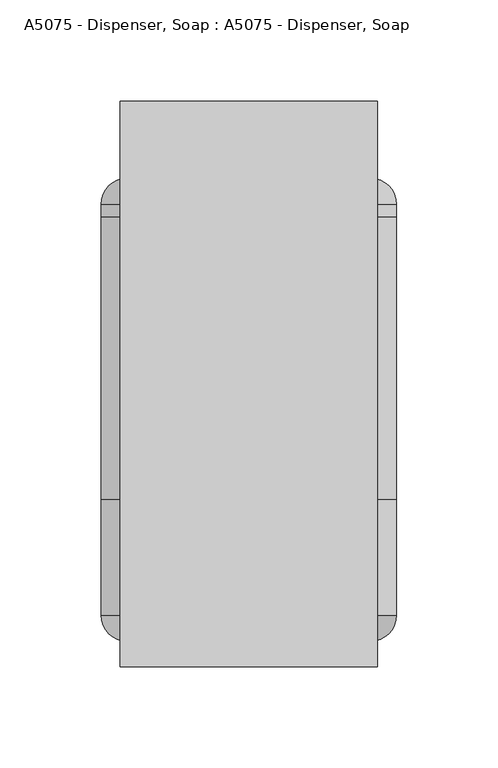
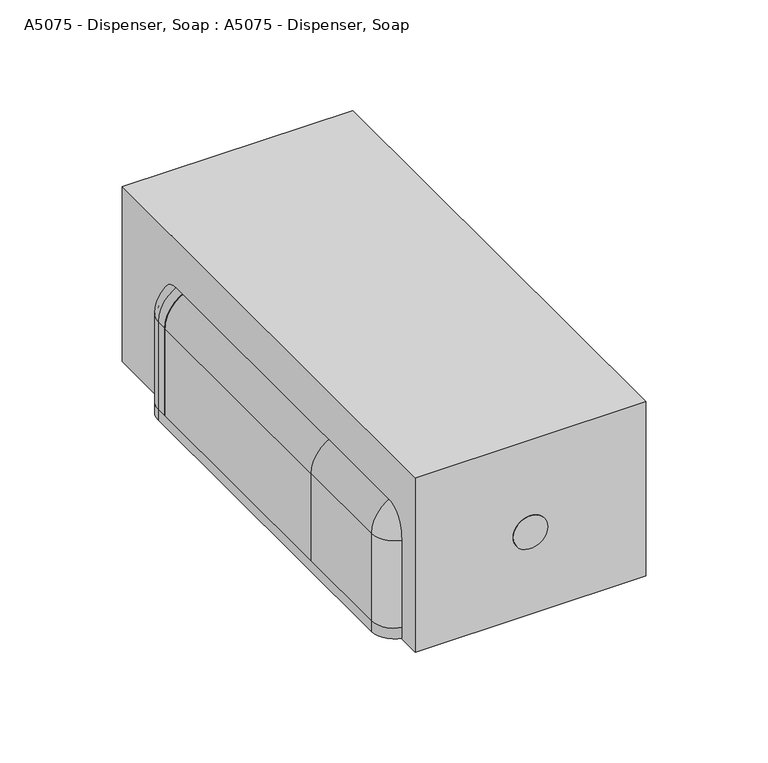
"""IFC4 building model written with IfcOpenShell, lengths in millimetres: proxy geometry, A5075 - Dispenser, Soap : A5075 - Dispenser, Soap."""

from ifc_helpers import new_model, si_unit, point, frame, frame_2d, origin, origin_with_axes, place, context, project, spatial, polyline, circle_curve, ellipse_curve, trimmed, segment, composite_curve, outline, extrude, source, transform, mapped, element, save
from ifc_brep_helpers import plane_surface, cylinder_surface, revolved_surface, advanced_brep


def a5075_dispenser_soap_a5075_dispenser_soap_4b3b6f7a(model_context):
    return source(origin(), model_context, "Body", "SolidModel", [
        advanced_brep(
        [(-73.025, 25.4, 6.35), (-73.025, 82.55, 6.35), (-71.4375, 82.55, 6.35), (-71.4375, 25.4, 6.35), (-60.325, 14.2875, 6.35), (-60.325, 12.7, 6.35), (-73.025, 25.4, 57.15), (-73.025, 82.55, 57.15), (-53.975, 82.55, 76.2), (53.975, 82.55, 76.2), (73.025, 82.55, 57.15), (73.025, 82.55, 6.35), (71.4375, 82.55, 6.35), (71.4375, 82.55, 57.15), (53.975, 82.55, 74.6125), (-53.975, 82.55, 74.6125), (-71.4375, 82.55, 57.15), (-71.4375, 25.4, 57.15), (-60.325, 14.2875, 57.15), (-60.325, 12.7, 57.15), (-53.975, 25.4, 76.2), (-53.975, 25.4, 74.6125), (-53.975, 14.2875, 63.5), (-53.975, 12.7, 63.5), (53.975, 25.4, 76.2), (53.975, 25.4, 74.6125), (53.975, 14.2875, 63.5), (53.975, 12.7, 63.5), (73.025, 25.4, 57.15), (71.4375, 25.4, 57.15), (60.325, 14.2875, 57.15), (60.325, 12.7, 57.15), (73.025, 25.4, 6.35), (60.325, 12.7, 6.35), (60.325, 14.2875, 6.35), (71.4375, 25.4, 6.35)],
        [
            (0, 1),
            (1, 2),
            (2, 3),
            (3, 4, circle_curve(frame((-60.325, 25.4, 6.35), z_axis=(0.0, 0.0, 1.0), x_axis=(1.0, 0.0, 0.0)), 11.1125)),
            (4, 5),
            (5, 0, circle_curve(frame((-60.325, 25.4, 6.35), z_axis=(0.0, 0.0, -1.0), x_axis=(1.0, 0.0, 0.0)), 12.7)),
            (0, 6),
            (6, 7),
            (7, 1),
            (7, 8, circle_curve(frame((-53.975, 82.55, 57.15), z_axis=(0.0, 1.0, 0.0), x_axis=(-1.0, 0.0, 0.0)), 19.05)),
            (8, 9),
            (9, 10, circle_curve(frame((53.975, 82.55, 57.15), z_axis=(0.0, 1.0, 0.0), x_axis=(0.0, 0.0, 1.0)), 19.05)),
            (10, 11),
            (11, 12),
            (12, 13),
            (13, 14, circle_curve(frame((53.975, 82.55, 57.15), z_axis=(0.0, -1.0, 0.0), x_axis=(0.0, 0.0, 1.0)), 17.4625)),
            (14, 15),
            (15, 16, circle_curve(frame((-53.975, 82.55, 57.15), z_axis=(0.0, -1.0, 0.0), x_axis=(-1.0, 0.0, 0.0)), 17.4625)),
            (16, 2),
            (16, 17),
            (17, 3),
            (17, 18, circle_curve(frame((-60.325, 25.4, 57.15), z_axis=(0.0, 0.0, 1.0), x_axis=(1.0, 0.0, 0.0)), 11.1125)),
            (18, 4),
            (18, 19),
            (19, 5),
            (19, 6, circle_curve(frame((-60.325, 25.4, 57.15), z_axis=(0.0, 0.0, -1.0), x_axis=(1.0, 0.0, 0.0)), 12.7)),
            (6, 20, circle_curve(frame((-53.975, 25.4, 57.15), z_axis=(0.0, 1.0, 0.0), x_axis=(-1.0, 0.0, 0.0)), 19.05)),
            (20, 8),
            (21, 17, circle_curve(frame((-53.975, 25.4, 57.15), z_axis=(0.0, -1.0, 0.0), x_axis=(-1.0, 0.0, 0.0)), 17.4625)),
            (15, 21),
            (22, 18, circle_curve(frame((-53.975, 14.2875, 57.15), z_axis=(0.0, -1.0, 0.0), x_axis=(-1.0, 0.0, 0.0)), 6.35)),
            (21, 22, circle_curve(frame((-53.975, 25.4, 63.5), z_axis=(1.0, 0.0, 0.0), x_axis=(0.0, 0.0, -1.0)), 11.1125)),
            (23, 19, circle_curve(frame((-53.975, 12.7, 57.15), z_axis=(0.0, -1.0, 0.0), x_axis=(-1.0, 0.0, 0.0)), 6.35)),
            (22, 23),
            (23, 20, circle_curve(frame((-53.975, 25.4, 63.5), z_axis=(-1.0, 0.0, 0.0), x_axis=(0.0, 0.0, -1.0)), 12.7)),
            (20, 24),
            (24, 9),
            (14, 25),
            (25, 21),
            (25, 26, circle_curve(frame((53.975, 25.4, 63.5), z_axis=(1.0, 0.0, 0.0), x_axis=(0.0, 0.0, -1.0)), 11.1125)),
            (26, 22),
            (26, 27),
            (27, 23),
            (27, 24, circle_curve(frame((53.975, 25.4, 63.5), z_axis=(-1.0, 0.0, 0.0), x_axis=(0.0, 0.0, -1.0)), 12.7)),
            (24, 28, circle_curve(frame((53.975, 25.4, 57.15), z_axis=(0.0, 1.0, 0.0), x_axis=(0.0, 0.0, 1.0)), 19.05)),
            (28, 10),
            (29, 25, circle_curve(frame((53.975, 25.4, 57.15), z_axis=(0.0, -1.0, 0.0), x_axis=(0.0, 0.0, 1.0)), 17.4625)),
            (13, 29),
            (30, 26, circle_curve(frame((53.975, 14.2875, 57.15), z_axis=(0.0, -1.0, 0.0), x_axis=(0.0, 0.0, 1.0)), 6.35)),
            (29, 30, circle_curve(frame((60.325, 25.4, 57.15), z_axis=(0.0, 0.0, -1.0), x_axis=(-1.0, 0.0, 0.0)), 11.1125)),
            (31, 27, circle_curve(frame((53.975, 12.7, 57.15), z_axis=(0.0, -1.0, 0.0), x_axis=(0.0, 0.0, 1.0)), 6.35)),
            (30, 31),
            (31, 28, circle_curve(frame((60.325, 25.4, 57.15), z_axis=(0.0, 0.0, 1.0), x_axis=(-1.0, 0.0, 0.0)), 12.7)),
            (32, 33, circle_curve(frame((60.325, 25.4, 6.35), z_axis=(0.0, 0.0, -1.0), x_axis=(-1.0, 0.0, 0.0)), 12.7)),
            (33, 34),
            (34, 35, circle_curve(frame((60.325, 25.4, 6.35), z_axis=(0.0, 0.0, 1.0), x_axis=(-1.0, 0.0, 0.0)), 11.1125)),
            (35, 12),
            (11, 32),
            (28, 32),
            (35, 29),
            (34, 30),
            (33, 31),
        ],
        [
            plane_surface(frame((-73.025, 12.7, 6.35), z_axis=(0.0, 0.0, -1.0), x_axis=(0.0, 1.0, 0.0))),
            plane_surface(frame((-73.025, 25.4, 6.35), z_axis=(-1.0, 0.0, 0.0), x_axis=(0.0, 0.0, 1.0))),
            plane_surface(frame((-73.025, 82.55, 6.35), z_axis=(0.0, 1.0, 0.0), x_axis=(0.0, 0.0, 1.0))),
            plane_surface(frame((-71.4375, 82.55, 6.35), z_axis=(1.0, 0.0, 0.0), x_axis=(0.0, 0.0, 1.0))),
            revolved_surface(polyline([(-49.212500000000006, 25.4, 57.15), (-49.212500000000006, 25.4, 6.35)]), (-60.325, 25.4, 6.35), (0.0, 0.0, 1.0)),
            plane_surface(frame((-60.325, 14.2875, 6.35), z_axis=(1.0, 0.0, 0.0), x_axis=(0.0, 0.0, 1.0))),
            cylinder_surface(frame((-60.325, 25.4, 6.35), z_axis=(0.0, 0.0, -1.0), x_axis=(1.0, 0.0, 0.0)), 12.7),
            cylinder_surface(frame((-53.975, 12.7, 57.15), z_axis=(0.0, 1.0, 0.0), x_axis=(-1.0, 0.0, 0.0)), 19.05),
            revolved_surface(polyline([(-71.4375, 82.55, 57.15), (-71.4375, 25.4, 57.15)]), (-53.975, 12.7, 57.15), (0.0, 1.0, 0.0)),
            revolved_surface(trimmed(ellipse_curve(frame((-60.325, 25.4, 57.15), z_axis=(0.0, 0.0, 1.0), x_axis=(1.0, 0.0, 0.0)), 11.1125, 11.1125), [point((-71.4375, 25.4, 57.15))], [point((-60.325, 14.2875, 57.15))], True, "CARTESIAN"), (-53.975, 12.7, 57.15), (0.0, 1.0, 0.0)),
            revolved_surface(polyline([(-60.325, 14.2875, 57.15), (-60.325, 12.7, 57.15)]), (-53.975, 12.7, 57.15), (0.0, 1.0, 0.0)),
            revolved_surface(trimmed(ellipse_curve(frame((-60.325, 25.4, 57.15), z_axis=(0.0, 0.0, -1.0), x_axis=(1.0, 0.0, 0.0)), 12.7, 12.7), [point((-60.325, 12.7, 57.15))], [point((-73.025, 25.4, 57.15))], True, "CARTESIAN"), (-53.975, 12.7, 57.15), (0.0, 1.0, 0.0)),
            plane_surface(frame((-53.975, 25.4, 76.2), z_axis=(0.0, 0.0, 1.0), x_axis=(1.0, 0.0, 0.0))),
            plane_surface(frame((-53.975, 82.55, 74.6125), z_axis=(0.0, 0.0, -1.0), x_axis=(1.0, 0.0, 0.0))),
            revolved_surface(polyline([(53.975, 25.4, 52.3875), (-53.975, 25.4, 52.3875)]), (-53.975, 25.4, 63.5), (1.0, 0.0, 0.0)),
            plane_surface(frame((-53.975, 14.2875, 63.5), z_axis=(0.0, 0.0, -1.0), x_axis=(1.0, 0.0, 0.0))),
            cylinder_surface(frame((-53.975, 25.4, 63.5), z_axis=(-1.0, 0.0, 0.0), x_axis=(0.0, 0.0, -1.0)), 12.7),
            cylinder_surface(frame((53.975, 12.7, 57.15), z_axis=(0.0, 1.0, 0.0), x_axis=(0.0, 0.0, 1.0)), 19.05),
            revolved_surface(polyline([(53.975, 82.55, 74.6125), (53.975, 25.4, 74.6125)]), (53.975, 12.7, 57.15), (0.0, 1.0, 0.0)),
            revolved_surface(trimmed(ellipse_curve(frame((53.975, 25.4, 63.5), z_axis=(1.0, 0.0, 0.0), x_axis=(0.0, 0.0, -1.0)), 11.1125, 11.1125), [point((53.975, 25.4, 74.6125))], [point((53.975, 14.2875, 63.5))], True, "CARTESIAN"), (53.975, 12.7, 57.15), (0.0, 1.0, 0.0)),
            revolved_surface(polyline([(53.975, 14.2875, 63.5), (53.975, 12.7, 63.5)]), (53.975, 12.7, 57.15), (0.0, 1.0, 0.0)),
            revolved_surface(trimmed(ellipse_curve(frame((53.975, 25.4, 63.5), z_axis=(-1.0, 0.0, 0.0), x_axis=(0.0, 0.0, -1.0)), 12.7, 12.7), [point((53.975, 12.7, 63.5))], [point((53.975, 25.4, 76.2))], True, "CARTESIAN"), (53.975, 12.7, 57.15), (0.0, 1.0, 0.0)),
            plane_surface(frame((73.025, 12.7, 6.35), z_axis=(0.0, 0.0, -1.0), x_axis=(0.0, 1.0, 0.0))),
            plane_surface(frame((73.025, 25.4, 57.15), z_axis=(1.0, 0.0, 0.0), x_axis=(0.0, 0.0, -1.0))),
            plane_surface(frame((71.4375, 82.55, 57.15), z_axis=(-1.0, 0.0, 0.0), x_axis=(0.0, 0.0, -1.0))),
            revolved_surface(polyline([(49.212500000000006, 25.4, 6.350000000000001), (49.212500000000006, 25.4, 57.15)]), (60.325, 25.4, 57.15), (0.0, 0.0, -1.0)),
            plane_surface(frame((60.325, 14.2875, 57.15), z_axis=(-1.0, 0.0, 0.0), x_axis=(0.0, 0.0, -1.0))),
            cylinder_surface(frame((60.325, 25.4, 57.15), z_axis=(0.0, 0.0, 1.0), x_axis=(-1.0, 0.0, 0.0)), 12.7),
        ],
        [
            (0, [[1, 2, 3, 4, 5, 6]]),
            (1, [[-1, 7, 8, 9]]),
            (2, [[-2, -9, 10, 11, 12, 13, 14, 15, 16, 17, 18, 19]]),
            (3, [[-3, -19, 20, 21]]),
            (4, [[-4, -21, 22, 23]]),
            (5, [[-5, -23, 24, 25]]),
            (6, [[-6, -25, 26, -7]]),
            (7, [[-10, -8, 27, 28]]),
            (8, [[29, -20, -18, 30]]),
            (9, [[31, -22, -29, 32]]),
            (10, [[33, -24, -31, 34]]),
            (11, [[-27, -26, -33, 35]]),
            (12, [[-28, 36, 37, -11]]),
            (13, [[-30, -17, 38, 39]]),
            (14, [[-32, -39, 40, 41]]),
            (15, [[-34, -41, 42, 43]]),
            (16, [[-35, -43, 44, -36]]),
            (17, [[-12, -37, 45, 46]]),
            (18, [[47, -38, -16, 48]]),
            (19, [[49, -40, -47, 50]]),
            (20, [[51, -42, -49, 52]]),
            (21, [[-45, -44, -51, 53]]),
            (22, [[54, 55, 56, 57, -14, 58]]),
            (23, [[-46, 59, -58, -13]]),
            (24, [[-48, -15, -57, 60]]),
            (25, [[-50, -60, -56, 61]]),
            (26, [[-52, -61, -55, 62]]),
            (27, [[-53, -62, -54, -59]]),
        ],
    ),
        advanced_brep(
        [(-73.025, 228.6, 6.35), (-60.325, 241.3, 6.35), (-60.325, 239.7125, 6.35), (-71.4375, 228.6, 6.35), (-71.4375, 222.25, 6.35), (-73.025, 222.25, 6.35), (-73.025, 228.6, 57.15), (-60.325, 241.3, 57.15), (-60.325, 239.7125, 57.15), (-71.4375, 228.6, 57.15), (-71.4375, 222.25, 57.15), (-53.975, 222.25, 74.6125), (53.975, 222.25, 74.6125), (71.4375, 222.25, 57.15), (71.4375, 222.25, 6.35), (73.025, 222.25, 6.35), (73.025, 222.25, 57.15), (53.975, 222.25, 76.2), (-53.975, 222.25, 76.2), (-73.025, 222.25, 57.15), (-53.975, 241.3, 63.5), (-53.975, 228.6, 76.2), (-53.975, 239.7125, 63.5), (-53.975, 228.6, 74.6125), (53.975, 228.6, 76.2), (53.975, 241.3, 63.5), (53.975, 239.7125, 63.5), (53.975, 228.6, 74.6125), (60.325, 241.3, 57.15), (73.025, 228.6, 57.15), (60.325, 239.7125, 57.15), (71.4375, 228.6, 57.15), (73.025, 228.6, 6.35), (71.4375, 228.6, 6.35), (60.325, 239.7125, 6.35), (60.325, 241.3, 6.35)],
        [
            (0, 1, circle_curve(frame((-60.325, 228.6, 6.35), z_axis=(0.0, 0.0, -1.0), x_axis=(1.0, 0.0, 0.0)), 12.7)),
            (1, 2),
            (2, 3, circle_curve(frame((-60.325, 228.6, 6.35), z_axis=(0.0, 0.0, 1.0), x_axis=(1.0, 0.0, 0.0)), 11.1125)),
            (3, 4),
            (4, 5),
            (5, 0),
            (0, 6),
            (6, 7, circle_curve(frame((-60.325, 228.6, 57.15), z_axis=(0.0, 0.0, -1.0), x_axis=(1.0, 0.0, 0.0)), 12.7)),
            (7, 1),
            (7, 8),
            (8, 2),
            (8, 9, circle_curve(frame((-60.325, 228.6, 57.15), z_axis=(0.0, 0.0, 1.0), x_axis=(1.0, 0.0, 0.0)), 11.1125)),
            (9, 3),
            (9, 10),
            (10, 4),
            (10, 11, circle_curve(frame((-53.975, 222.25, 57.15), z_axis=(0.0, 1.0, 0.0), x_axis=(-1.0, 0.0, 0.0)), 17.4625)),
            (11, 12),
            (12, 13, circle_curve(frame((53.975, 222.25, 57.15), z_axis=(0.0, 1.0, 0.0), x_axis=(0.0, 0.0, 1.0)), 17.4625)),
            (13, 14),
            (14, 15),
            (15, 16),
            (16, 17, circle_curve(frame((53.975, 222.25, 57.15), z_axis=(0.0, -1.0, 0.0), x_axis=(0.0, 0.0, 1.0)), 19.05)),
            (17, 18),
            (18, 19, circle_curve(frame((-53.975, 222.25, 57.15), z_axis=(0.0, -1.0, 0.0), x_axis=(-1.0, 0.0, 0.0)), 19.05)),
            (19, 5),
            (19, 6),
            (20, 7, circle_curve(frame((-53.975, 241.3, 57.15), z_axis=(0.0, -1.0, 0.0), x_axis=(-1.0, 0.0, 0.0)), 6.35)),
            (6, 21, circle_curve(frame((-53.975, 228.6, 57.15), z_axis=(0.0, 1.0, 0.0), x_axis=(-1.0, 0.0, 0.0)), 19.05)),
            (21, 20, circle_curve(frame((-53.975, 228.6, 63.5), z_axis=(-1.0, 0.0, 0.0), x_axis=(0.0, 0.0, -1.0)), 12.7)),
            (22, 8, circle_curve(frame((-53.975, 239.7125, 57.15), z_axis=(0.0, -1.0, 0.0), x_axis=(-1.0, 0.0, 0.0)), 6.35)),
            (20, 22),
            (23, 9, circle_curve(frame((-53.975, 228.6, 57.15), z_axis=(0.0, -1.0, 0.0), x_axis=(-1.0, 0.0, 0.0)), 17.4625)),
            (22, 23, circle_curve(frame((-53.975, 228.6, 63.5), z_axis=(1.0, 0.0, 0.0), x_axis=(0.0, 0.0, -1.0)), 11.1125)),
            (23, 11),
            (18, 21),
            (21, 24),
            (24, 25, circle_curve(frame((53.975, 228.6, 63.5), z_axis=(-1.0, 0.0, 0.0), x_axis=(0.0, 0.0, -1.0)), 12.7)),
            (25, 20),
            (25, 26),
            (26, 22),
            (26, 27, circle_curve(frame((53.975, 228.6, 63.5), z_axis=(1.0, 0.0, 0.0), x_axis=(0.0, 0.0, -1.0)), 11.1125)),
            (27, 23),
            (27, 12),
            (17, 24),
            (28, 25, circle_curve(frame((53.975, 241.3, 57.15), z_axis=(0.0, -1.0, 0.0), x_axis=(0.0, 0.0, 1.0)), 6.35)),
            (24, 29, circle_curve(frame((53.975, 228.6, 57.15), z_axis=(0.0, 1.0, 0.0), x_axis=(0.0, 0.0, 1.0)), 19.05)),
            (29, 28, circle_curve(frame((60.325, 228.6, 57.15), z_axis=(0.0, 0.0, 1.0), x_axis=(-1.0, 0.0, 0.0)), 12.7)),
            (30, 26, circle_curve(frame((53.975, 239.7125, 57.15), z_axis=(0.0, -1.0, 0.0), x_axis=(0.0, 0.0, 1.0)), 6.35)),
            (28, 30),
            (31, 27, circle_curve(frame((53.975, 228.6, 57.15), z_axis=(0.0, -1.0, 0.0), x_axis=(0.0, 0.0, 1.0)), 17.4625)),
            (30, 31, circle_curve(frame((60.325, 228.6, 57.15), z_axis=(0.0, 0.0, -1.0), x_axis=(-1.0, 0.0, 0.0)), 11.1125)),
            (31, 13),
            (16, 29),
            (32, 15),
            (14, 33),
            (33, 34, circle_curve(frame((60.325, 228.6, 6.35), z_axis=(0.0, 0.0, 1.0), x_axis=(-1.0, 0.0, 0.0)), 11.1125)),
            (34, 35),
            (35, 32, circle_curve(frame((60.325, 228.6, 6.35), z_axis=(0.0, 0.0, -1.0), x_axis=(-1.0, 0.0, 0.0)), 12.7)),
            (29, 32),
            (35, 28),
            (34, 30),
            (33, 31),
        ],
        [
            plane_surface(frame((-73.025, 241.3, 6.35), z_axis=(0.0, 0.0, -1.0), x_axis=(0.0, 1.0, 0.0))),
            cylinder_surface(frame((-60.325, 228.6, 6.35), z_axis=(0.0, 0.0, -1.0), x_axis=(1.0, 0.0, 0.0)), 12.7),
            plane_surface(frame((-60.325, 241.3, 6.35), z_axis=(1.0, 0.0, 0.0), x_axis=(0.0, 0.0, 1.0))),
            revolved_surface(polyline([(-49.212500000000006, 228.6, 57.15), (-49.212500000000006, 228.6, 6.35)]), (-60.325, 228.6, 6.35), (0.0, 0.0, 1.0)),
            plane_surface(frame((-71.4375, 228.6, 6.35), z_axis=(1.0, 0.0, 0.0), x_axis=(0.0, 0.0, 1.0))),
            plane_surface(frame((-71.4375, 222.25, 6.35), z_axis=(0.0, -1.0, 0.0), x_axis=(0.0, 0.0, 1.0))),
            plane_surface(frame((-73.025, 222.25, 6.35), z_axis=(-1.0, 0.0, 0.0), x_axis=(0.0, 0.0, 1.0))),
            revolved_surface(trimmed(ellipse_curve(frame((-60.325, 228.6, 57.15), z_axis=(0.0, 0.0, -1.0), x_axis=(1.0, 0.0, 0.0)), 12.7, 12.7), [point((-73.025, 228.6, 57.15))], [point((-60.325, 241.3, 57.15))], True, "CARTESIAN"), (-53.975, 241.3, 57.15), (0.0, 1.0, 0.0)),
            revolved_surface(polyline([(-60.325, 241.3, 57.15), (-60.325, 239.7125, 57.15)]), (-53.975, 241.3, 57.15), (0.0, 1.0, 0.0)),
            revolved_surface(trimmed(ellipse_curve(frame((-60.325, 228.6, 57.15), z_axis=(0.0, 0.0, 1.0), x_axis=(1.0, 0.0, 0.0)), 11.1125, 11.1125), [point((-60.325, 239.7125, 57.15))], [point((-71.4375, 228.6, 57.15))], True, "CARTESIAN"), (-53.975, 241.3, 57.15), (0.0, 1.0, 0.0)),
            revolved_surface(polyline([(-71.4375, 228.6, 57.15), (-71.4375, 222.25, 57.15)]), (-53.975, 241.3, 57.15), (0.0, 1.0, 0.0)),
            cylinder_surface(frame((-53.975, 241.3, 57.15), z_axis=(0.0, 1.0, 0.0), x_axis=(-1.0, 0.0, 0.0)), 19.05),
            cylinder_surface(frame((-53.975, 228.6, 63.5), z_axis=(-1.0, 0.0, 0.0), x_axis=(0.0, 0.0, -1.0)), 12.7),
            plane_surface(frame((-53.975, 241.3, 63.5), z_axis=(0.0, 0.0, -1.0), x_axis=(1.0, 0.0, 0.0))),
            revolved_surface(polyline([(53.975, 228.6, 52.3875), (-53.975, 228.6, 52.3875)]), (-53.975, 228.6, 63.5), (1.0, 0.0, 0.0)),
            plane_surface(frame((-53.975, 228.6, 74.6125), z_axis=(0.0, 0.0, -1.0), x_axis=(1.0, 0.0, 0.0))),
            plane_surface(frame((-53.975, 222.25, 76.2), z_axis=(0.0, 0.0, 1.0), x_axis=(1.0, 0.0, 0.0))),
            revolved_surface(trimmed(ellipse_curve(frame((53.975, 228.6, 63.5), z_axis=(-1.0, 0.0, 0.0), x_axis=(0.0, 0.0, -1.0)), 12.7, 12.7), [point((53.975, 228.6, 76.2))], [point((53.975, 241.3, 63.5))], True, "CARTESIAN"), (53.975, 241.3, 57.15), (0.0, 1.0, 0.0)),
            revolved_surface(polyline([(53.975, 241.3, 63.5), (53.975, 239.7125, 63.5)]), (53.975, 241.3, 57.15), (0.0, 1.0, 0.0)),
            revolved_surface(trimmed(ellipse_curve(frame((53.975, 228.6, 63.5), z_axis=(1.0, 0.0, 0.0), x_axis=(0.0, 0.0, -1.0)), 11.1125, 11.1125), [point((53.975, 239.7125, 63.5))], [point((53.975, 228.6, 74.6125))], True, "CARTESIAN"), (53.975, 241.3, 57.15), (0.0, 1.0, 0.0)),
            revolved_surface(polyline([(53.975, 228.6, 74.6125), (53.975, 222.25, 74.6125)]), (53.975, 241.3, 57.15), (0.0, 1.0, 0.0)),
            cylinder_surface(frame((53.975, 241.3, 57.15), z_axis=(0.0, 1.0, 0.0), x_axis=(0.0, 0.0, 1.0)), 19.05),
            plane_surface(frame((73.025, 241.3, 6.35), z_axis=(0.0, 0.0, -1.0), x_axis=(0.0, 1.0, 0.0))),
            cylinder_surface(frame((60.325, 228.6, 57.15), z_axis=(0.0, 0.0, 1.0), x_axis=(-1.0, 0.0, 0.0)), 12.7),
            plane_surface(frame((60.325, 241.3, 57.15), z_axis=(-1.0, 0.0, 0.0), x_axis=(0.0, 0.0, -1.0))),
            revolved_surface(polyline([(49.212500000000006, 228.6, 6.350000000000001), (49.212500000000006, 228.6, 57.15)]), (60.325, 228.6, 57.15), (0.0, 0.0, -1.0)),
            plane_surface(frame((71.4375, 228.6, 57.15), z_axis=(-1.0, 0.0, 0.0), x_axis=(0.0, 0.0, -1.0))),
            plane_surface(frame((73.025, 222.25, 57.15), z_axis=(1.0, 0.0, 0.0), x_axis=(0.0, 0.0, -1.0))),
        ],
        [
            (0, [[1, 2, 3, 4, 5, 6]]),
            (1, [[-1, 7, 8, 9]]),
            (2, [[-2, -9, 10, 11]]),
            (3, [[-3, -11, 12, 13]]),
            (4, [[-4, -13, 14, 15]]),
            (5, [[-5, -15, 16, 17, 18, 19, 20, 21, 22, 23, 24, 25]]),
            (6, [[-6, -25, 26, -7]]),
            (7, [[27, -8, 28, 29]]),
            (8, [[30, -10, -27, 31]]),
            (9, [[32, -12, -30, 33]]),
            (10, [[-16, -14, -32, 34]]),
            (11, [[-28, -26, -24, 35]]),
            (12, [[-29, 36, 37, 38]]),
            (13, [[-31, -38, 39, 40]]),
            (14, [[-33, -40, 41, 42]]),
            (15, [[-34, -42, 43, -17]]),
            (16, [[-35, -23, 44, -36]]),
            (17, [[45, -37, 46, 47]]),
            (18, [[48, -39, -45, 49]]),
            (19, [[50, -41, -48, 51]]),
            (20, [[-18, -43, -50, 52]]),
            (21, [[-46, -44, -22, 53]]),
            (22, [[54, -20, 55, 56, 57, 58]]),
            (23, [[-47, 59, -58, 60]]),
            (24, [[-49, -60, -57, 61]]),
            (25, [[-51, -61, -56, 62]]),
            (26, [[-52, -62, -55, -19]]),
            (27, [[-53, -21, -54, -59]]),
        ],
    ),
        extrude(outline(composite_curve([segment(polyline([(57.15, -73.025), (6.35, -73.025), (6.35, -71.4375), (57.15, -71.4375)]), True, "CONTINUOUS"), segment(trimmed(circle_curve(frame_2d((57.15, -53.975)), 17.4625), [point((57.15, -71.4375))], [point((74.6125, -53.975))], True, "CARTESIAN"), True, "CONTINUOUS"), segment(polyline([(74.6125, -53.975), (74.6125, 53.975)]), True, "CONTINUOUS"), segment(trimmed(circle_curve(frame_2d((57.15, 53.975)), 17.4625), [point((74.6125, 53.975))], [point((57.15, 71.4375))], True, "CARTESIAN"), True, "CONTINUOUS"), segment(polyline([(57.15, 71.4375), (6.35, 71.4375), (6.35, 73.025), (57.15, 73.025)]), True, "CONTINUOUS"), segment(trimmed(circle_curve(frame_2d((57.15, 53.975)), 19.05), [point((57.15, 73.025))], [point((76.2, 53.975))], False, "CARTESIAN"), True, "CONTINUOUS"), segment(polyline([(76.2, 53.975), (76.2, -53.975)]), True, "CONTINUOUS"), segment(trimmed(circle_curve(frame_2d((57.15, -53.975)), 19.05), [point((76.2, -53.975))], [point((57.15, -73.025))], False, "CARTESIAN"), True, "CONTINUOUS")], self_intersect=False)), frame((0.0, 82.55, 0.0), z_axis=(0.0, 1.0, 0.0), x_axis=(0.0, 0.0, 1.0)), (0.0, 0.0, 1.0), 139.7),
        extrude(outline(composite_curve([segment(polyline([(74.6125, 53.975), (74.6125, -53.975)]), True, "CONTINUOUS"), segment(trimmed(circle_curve(frame_2d((57.15, -53.975)), 17.4625), [point((74.6125, -53.975))], [point((57.15, -71.4375))], False, "CARTESIAN"), True, "CONTINUOUS"), segment(polyline([(57.15, -71.4375), (6.35, -71.4375), (6.35, 71.4375), (57.15, 71.4375)]), True, "CONTINUOUS"), segment(trimmed(circle_curve(frame_2d((57.15, 53.975)), 17.4625), [point((57.15, 71.4375))], [point((74.6125, 53.975))], False, "CARTESIAN"), True, "CONTINUOUS")], self_intersect=False)), frame((0.0, 82.55, 0.0), z_axis=(0.0, 1.0, 0.0), x_axis=(0.0, 0.0, 1.0)), (0.0, 0.0, 1.0), 101.8530988),
        extrude(outline(composite_curve([segment(trimmed(circle_curve(frame_2d((47.625, 0.0)), 9.525), [point((47.625, -9.525))], [point((47.625, 9.525))], False, "CARTESIAN"), True, "CONTINUOUS"), segment(trimmed(circle_curve(frame_2d((47.625, 0.0)), 9.525), [point((47.625, 9.525))], [point((47.625, -9.525))], False, "CARTESIAN"), True, "CONTINUOUS")], self_intersect=False)), frame((0.0, 0.0, 0.0), z_axis=(0.0, 1.0, 0.0), x_axis=(0.0, 0.0, 1.0)), (0.0, 0.0, 1.0), 12.7),
        extrude(outline(composite_curve([segment(polyline([(-9.525, 50.8), (9.525, 50.8)]), True, "CONTINUOUS"), segment(trimmed(circle_curve(frame_2d((9.525, 41.275)), 9.525), [point((9.525, 50.8))], [point((9.525, 31.75))], False, "CARTESIAN"), True, "CONTINUOUS"), segment(polyline([(9.525, 31.75), (-9.525, 31.75)]), True, "CONTINUOUS"), segment(trimmed(circle_curve(frame_2d((-9.525, 41.275)), 9.525), [point((-9.525, 31.75))], [point((-9.525, 50.8))], False, "CARTESIAN"), True, "CONTINUOUS")], self_intersect=False)), frame((0.0, 0.0, 76.2), z_axis=(0.0, 0.0, 1.0), x_axis=(1.0, 0.0, 0.0)), (0.0, 0.0, 1.0), 12.7),
        extrude(outline(composite_curve([segment(polyline([(6.35, -60.325), (6.35, 60.325), (57.15, 60.325)]), True, "CONTINUOUS"), segment(trimmed(circle_curve(frame_2d((57.15, 53.975)), 6.35), [point((57.15, 60.325))], [point((63.5, 53.975))], False, "CARTESIAN"), True, "CONTINUOUS"), segment(polyline([(63.5, 53.975), (63.5, -53.975)]), True, "CONTINUOUS"), segment(trimmed(circle_curve(frame_2d((57.15, -53.975)), 6.35), [point((63.5, -53.975))], [point((57.15, -60.325))], False, "CARTESIAN"), True, "CONTINUOUS"), segment(polyline([(57.15, -60.325), (6.35, -60.325)]), True, "CONTINUOUS")], self_intersect=False)), frame((0.0, 12.7, 0.0), z_axis=(0.0, 1.0, 0.0), x_axis=(0.0, 0.0, 1.0)), (0.0, 0.0, 1.0), 1.5875),
        extrude(outline(composite_curve([segment(polyline([(-60.325, 241.3), (60.325, 241.3)]), True, "CONTINUOUS"), segment(trimmed(circle_curve(frame_2d((60.325, 228.6)), 12.7), [point((60.325, 241.3))], [point((73.025, 228.6))], False, "CARTESIAN"), True, "CONTINUOUS"), segment(polyline([(73.025, 228.6), (73.025, 25.4)]), True, "CONTINUOUS"), segment(trimmed(circle_curve(frame_2d((60.325, 25.4)), 12.7), [point((73.025, 25.4))], [point((60.325, 12.7))], False, "CARTESIAN"), True, "CONTINUOUS"), segment(polyline([(60.325, 12.7), (-60.325, 12.7)]), True, "CONTINUOUS"), segment(trimmed(circle_curve(frame_2d((-60.325, 25.4)), 12.7), [point((-60.325, 12.7))], [point((-73.025, 25.4))], False, "CARTESIAN"), True, "CONTINUOUS"), segment(polyline([(-73.025, 25.4), (-73.025, 228.6)]), True, "CONTINUOUS"), segment(trimmed(circle_curve(frame_2d((-60.325, 228.6)), 12.7), [point((-73.025, 228.6))], [point((-60.325, 241.3))], False, "CARTESIAN"), True, "CONTINUOUS")], self_intersect=False)), origin_with_axes(), (0.0, 0.0, 1.0), 6.35),
        extrude(outline(polyline([(63.5, 279.4), (63.5, 0.0), (-63.5, 0.0), (-63.5, 279.4), (63.5, 279.4)])), origin_with_axes(), (0.0, 0.0, 1.0), 101.6),
        extrude(outline(composite_curve([segment(polyline([(6.35, -60.325), (6.35, 60.325), (57.15, 60.325)]), True, "CONTINUOUS"), segment(trimmed(circle_curve(frame_2d((57.15, 53.975)), 6.35), [point((57.15, 60.325))], [point((63.5, 53.975))], False, "CARTESIAN"), True, "CONTINUOUS"), segment(polyline([(63.5, 53.975), (63.5, -53.975)]), True, "CONTINUOUS"), segment(trimmed(circle_curve(frame_2d((57.15, -53.975)), 6.35), [point((63.5, -53.975))], [point((57.15, -60.325))], False, "CARTESIAN"), True, "CONTINUOUS"), segment(polyline([(57.15, -60.325), (6.35, -60.325)]), True, "CONTINUOUS")], self_intersect=False)), frame((0.0, 239.7125, 0.0), z_axis=(0.0, 1.0, 0.0), x_axis=(0.0, 0.0, 1.0)), (0.0, 0.0, 1.0), 1.5875),
    ])


if __name__ == "__main__":
    model = new_model("IFC4")
    model_context = context("Model", 3, world=origin())
    ifc_project = project(units=[si_unit("LENGTHUNIT", "METRE", prefix="MILLI")], contexts=[model_context])
    site = spatial("IfcSite", under=ifc_project)
    building = spatial("IfcBuilding", under=site)
    placement = place(None, origin())
    a5075_dispenser_soap_a5075_dispenser_soap_shape = a5075_dispenser_soap_a5075_dispenser_soap_4b3b6f7a(model_context)
    element("IfcBuildingElementProxy", 1, Name="A5075 - Dispenser, Soap : A5075 - Dispenser, Soap", ObjectType="A5075 - Dispenser, Soap : A5075 - Dispenser, Soap", at=placement, inside=building, context=model_context, shape_type="MappedRepresentation", body=[
        mapped(a5075_dispenser_soap_a5075_dispenser_soap_shape, transform((0.0, 0.0, 0.0), x_axis=(1.0, 0.0, 0.0), y_axis=(0.0, 1.0, 0.0), z_axis=(0.0, 0.0, 1.0))),
    ])
    save(model, "model.ifc")

# Revit data of these elements
# Type "A5075 - Dispenser, Soap : A5075 - Dispenser, Soap"
#   Watts2 = "0"
#   Watts1 = "0"
#   Unit_Issue = "EA"
#   UTIL_6_Misc = "-"
#   UTIL_5_NonMedGas = "-"
#   UTIL_4_MiscGas = "-"
#   UTIL_3_MedGas = "-"
#   UTIL_2_Elec = "-"
#   UTIL_1_WaterDrain = "-"
#   Nomenclature = "Dispenser, Soap, Disposable"
#   NSN = "4510"
#   Location [instance default] = ""
#   JSN = "A5075"
#   Fund_Source_VA = "-"
#   Fund_Source_Navy = "-"
#   Fund_Source_Army = "-"
#   Fund_Source_AF = "-"
#   ELEC_Volts2 = "0"
#   ELEC_Volts1 = "0"
#   ELEC_Phase2 = "0"
#   ELEC_Phase1 = "0"
#   ELEC_HertzSwitch = "0"
#   ELEC_HertzDependent = "0"
#   ELEC_Hertz = "0"
#   ELEC_Amps2 = "0"
#   ELEC_Amps1 = "0"
#   DetailDescription = "Disposable soap dispenser. One-handed dispensing operation. Designed to accommodate disposable soap cartridge and valve."
#   CAT_VA = "C"
#   CAT_Navy = "C"
#   CAT_IHS = "-"
#   CAT_Army = "C"
#   CAT_AF = "C"
#   BTUperhour = "0"
#   Weight_IP = 3
#   Default Elevation = 3' - 6"
#   DIM_Width_IP = 0' - 5"
#   DIM_Height_IP = 0' - 11"
#   DIM_Depth_IP = 0' - 4"
#   Assembly Code = ""
# Element 1 (IfcBuildingElementProxy, "A5075 - Dispenser, Soap : A5075 - Dispenser, Soap")
#   Location = "TRET3"
#   Materials on its faces: "White Paint", "Glass", "EquipSpace"
# Materials
#   "White Paint": class "Unassigned", colour RGB 249 249 249, transparency 0
#   "Glass": class "Glass", colour RGB 0 128 192, transparency 0.75
#   "EquipSpace": class "Unassigned", colour RGB 221 217 195, transparency 0.5
